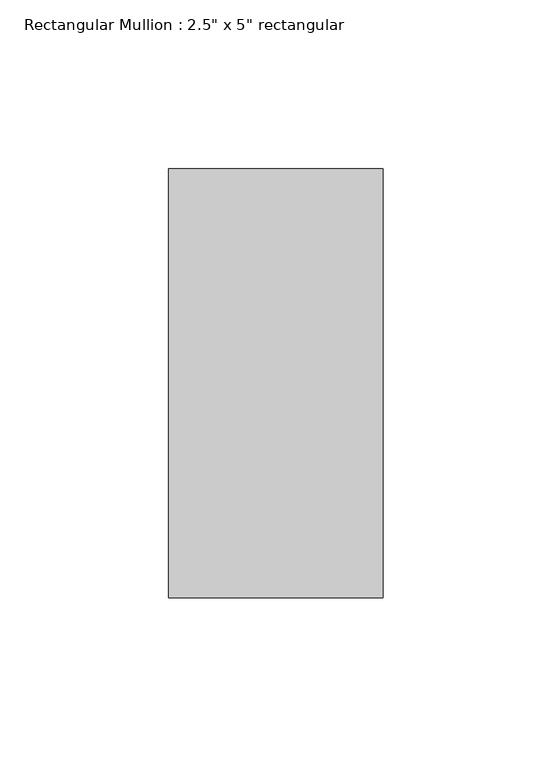
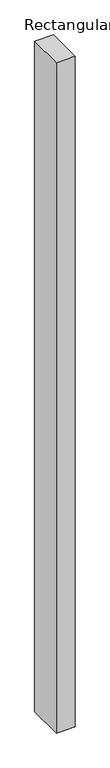
"""IFC4 building model written with IfcOpenShell, lengths in millimetres: member geometry."""

import ifcopenshell
import ifcopenshell.guid

model = None  # the IFC model being written
_history = None  # IfcOwnerHistory: only IFC2X3 demands one
_inside = {}  # id of a spatial element -> (the spatial element, [elements in it])
_under = {}  # id of a project, library or spatial element -> (it, [spatial elements below it])
_declared = {}  # id of a project -> (the project, [libraries it declares])
_typed = {}  # id of a type object -> (the type object, [elements of that type])
_made_of = {}  # id of a material, layer set ... -> (it, [elements and type objects made of it])


def new_model(schema):
    """Start an empty IFC model of exactly this schema.

    Asked for "IFC4X3", IfcOpenShell would pick the latest addendum, in which some entities
    have other attributes; the version numbers below select the first issue.
    IFC2X3 requires an IfcOwnerHistory on every rooted entity: one is made here for all.
    """
    global model, _history
    if schema == "IFC4X3":
        model = ifcopenshell.file(schema_version=(4, 3, 0, 0))
    else:
        model = ifcopenshell.file(schema=schema)
    _inside.clear()
    _under.clear()
    _declared.clear()
    _typed.clear()
    _made_of.clear()
    _history = None
    if model.schema == "IFC2X3":
        org = make("IfcOrganization", Name="unknown")
        user = make(
            "IfcPersonAndOrganization",
            ThePerson=make("IfcPerson", FamilyName="unknown"),
            TheOrganization=org,
        )
        app = make(
            "IfcApplication",
            ApplicationDeveloper=org,
            Version="unknown",
            ApplicationFullName="unknown",
            ApplicationIdentifier="unknown",
        )
        _history = make(
            "IfcOwnerHistory",
            OwningUser=user,
            OwningApplication=app,
            ChangeAction="ADDED",
            CreationDate=0,
        )
    return model


def make(cls, **values):
    """One entity of the class cls with the attributes given. An attribute that is None is left unset."""
    return model.create_entity(
        cls, **{name: value for name, value in values.items() if value is not None}
    )


def rooted(cls, **values):
    """An entity with a GlobalId (a new one), such as an element, a storey or a relation."""
    return make(cls, GlobalId=ifcopenshell.guid.new(), OwnerHistory=_history, **values)


def si_unit(unit_type, name, prefix=None):
    """IfcSIUnit, for example si_unit("LENGTHUNIT", "METRE", prefix="MILLI")."""
    return make("IfcSIUnit", UnitType=unit_type, Prefix=prefix, Name=name)


def assignment(units):
    """IfcUnitAssignment: the units of a project."""
    return None if units is None else make("IfcUnitAssignment", Units=units)


def point(xyz):
    """IfcCartesianPoint."""
    return None if xyz is None else make("IfcCartesianPoint", Coordinates=xyz)


def direction(xyz):
    """IfcDirection."""
    return None if xyz is None else make("IfcDirection", DirectionRatios=xyz)


def frame(location, z_axis=None, x_axis=None):
    """IfcAxis2Placement3D, a coordinate frame: its origin and axes. An axis left out is left unset."""
    return make(
        "IfcAxis2Placement3D",
        Location=point(location),
        Axis=direction(z_axis),
        RefDirection=direction(x_axis),
    )


def origin():
    """The frame at (0, 0, 0) with its axes left unset."""
    return frame((0.0, 0.0, 0.0))


def place(relative_to, where):
    """IfcLocalPlacement: puts the frame where relative to a parent placement (None: the world)."""
    return make(
        "IfcLocalPlacement", PlacementRelTo=relative_to, RelativePlacement=where
    )


def context(
    kind, dimensions, precision=None, world=None, true_north=None, identifier=None
):
    """IfcGeometricRepresentationContext, for example the 3D "Model" context."""
    return make(
        "IfcGeometricRepresentationContext",
        ContextIdentifier=identifier,
        ContextType=kind,
        CoordinateSpaceDimension=dimensions,
        Precision=precision,
        WorldCoordinateSystem=world,
        TrueNorth=true_north,
    )


def project(units=None, contexts=None):
    """IfcProject with its units and contexts."""
    return rooted(
        "IfcProject",
        Name="project",
        RepresentationContexts=contexts,
        UnitsInContext=assignment(units),
    )


def spatial(cls, under=None, at=None, **own):
    """A site, building, storey or space (cls), placed at a placement, below another one or the project."""
    s = rooted(cls, ObjectPlacement=at, **own)
    if under is not None:
        _under.setdefault(under.id(), (under, []))[1].append(s)
    return s


def polyline(points):
    """IfcPolyline through the points."""
    return make("IfcPolyline", Points=[point(p) for p in points])


def outline(outer, holes=None, kind="AREA"):
    """IfcArbitraryClosedProfileDef: a profile drawn as a closed curve; with holes, ...WithVoids."""
    if holes is None:
        return make("IfcArbitraryClosedProfileDef", ProfileType=kind, OuterCurve=outer)
    return make(
        "IfcArbitraryProfileDefWithVoids",
        ProfileType=kind,
        OuterCurve=outer,
        InnerCurves=holes,
    )


def extrude(swept, where, along, depth):
    """IfcExtrudedAreaSolid: the profile swept, set in the frame where, extruded along a direction by depth."""
    return make(
        "IfcExtrudedAreaSolid",
        SweptArea=swept,
        Position=where,
        ExtrudedDirection=direction(along),
        Depth=depth,
    )


def shape(context_of_items, identifier, shape_type, items):
    """IfcShapeRepresentation: the items that make up one representation, for example the "Body"."""
    return make(
        "IfcShapeRepresentation",
        ContextOfItems=context_of_items,
        RepresentationIdentifier=identifier,
        RepresentationType=shape_type,
        Items=items,
    )


def source(mapping_origin, context_of_items, identifier, shape_type, items):
    """IfcRepresentationMap: a shape defined once, which mapped items show again and again."""
    return make(
        "IfcRepresentationMap",
        MappingOrigin=mapping_origin,
        MappedRepresentation=shape(context_of_items, identifier, shape_type, items),
    )


def transform(
    local_origin,
    x_axis=None,
    y_axis=None,
    z_axis=None,
    scale=None,
    scale2=None,
    scale3=None,
    uniform=True,
):
    """IfcCartesianTransformationOperator3D, or its non-uniform kind. x_axis, y_axis, z_axis: its Axis1, 2, 3."""
    if uniform:
        return make(
            "IfcCartesianTransformationOperator3D",
            Axis1=direction(x_axis),
            Axis2=direction(y_axis),
            LocalOrigin=point(local_origin),
            Scale=scale,
            Axis3=direction(z_axis),
        )
    return make(
        "IfcCartesianTransformationOperator3DnonUniform",
        Axis1=direction(x_axis),
        Axis2=direction(y_axis),
        LocalOrigin=point(local_origin),
        Scale=scale,
        Axis3=direction(z_axis),
        Scale2=scale2,
        Scale3=scale3,
    )


def mapped(mapping_source, mapping_target):
    """IfcMappedItem: shows the shape of a source again, moved by a transform."""
    return make(
        "IfcMappedItem", MappingSource=mapping_source, MappingTarget=mapping_target
    )


def made_of(thing, what):
    """Note that an element or type object is made of a material, layer set ...; save() writes the relation."""
    if what is not None:
        _made_of.setdefault(what.id(), (what, []))[1].append(thing)
    return thing


def element(
    cls,
    number,
    at=None,
    inside=None,
    cuts=None,
    type_object=None,
    material=None,
    context=None,
    identifier="Body",
    shape_type=None,
    held_by="IfcProductDefinitionShape",
    body=None,
    shapes=None,
    **own,
):
    """One element of the class cls, such as IfcWall. Its Tag is "e" and its number.

    at: its placement. inside: the storey or other place that contains it. cuts: it is an
    opening in that element (IfcRelVoidsElement). A single representation is given by context,
    identifier, shape_type and body (its items); several are given by shapes. held_by: the class
    of the entity that holds the representations. save() writes the other relations.
    """
    e = rooted(cls, Tag="e%d" % number, ObjectPlacement=at, **own)
    if body is not None:
        shapes = [shape(context, identifier, shape_type, body)]
    if shapes is not None:
        e.Representation = make(held_by, Representations=shapes)
    if inside is not None:
        _inside.setdefault(inside.id(), (inside, []))[1].append(e)
    if cuts is not None:
        rooted(
            "IfcRelVoidsElement", RelatingBuildingElement=cuts, RelatedOpeningElement=e
        )
    if type_object is not None:
        _typed.setdefault(type_object.id(), (type_object, []))[1].append(e)
    return made_of(e, material)


def aggregate(whole, parts):
    """IfcRelAggregates: a whole, such as a stair, and the parts it consists of."""
    return rooted("IfcRelAggregates", RelatingObject=whole, RelatedObjects=parts)


def save(model, path):
    """Write the relations noted so far, then the file.

    IfcRelAggregates (storeys below a building ...), IfcRelContainedInSpatialStructure (elements
    in a storey), IfcRelDefinesByType, IfcRelAssociatesMaterial and IfcRelDeclares: one each for
    every whole, place, type object, material and project.
    """
    for whole, parts in _under.values():
        aggregate(whole, parts)
    for where, things in _inside.values():
        rooted(
            "IfcRelContainedInSpatialStructure",
            RelatedElements=things,
            RelatingStructure=where,
        )
    for kind, things in _typed.values():
        rooted("IfcRelDefinesByType", RelatedObjects=things, RelatingType=kind)
    for what, things in _made_of.values():
        rooted("IfcRelAssociatesMaterial", RelatedObjects=things, RelatingMaterial=what)
    for by, libraries in _declared.values():
        rooted("IfcRelDeclares", RelatingContext=by, RelatedDefinitions=libraries)
    model.write(path)


def member_5511fbbe(model_context):
    return source(origin(), model_context, "Body", "SweptSolid", [
        extrude(outline(polyline([(0.0, 63.5), (0.0, -63.5), (-63.5, -63.5), (-63.5, 63.5), (0.0, 63.5)])), frame((0.0, 0.0, -2398.3630718), z_axis=(0.0, 0.0, 1.0), x_axis=(1.0, 0.0, 0.0)), (0.0, 0.0, 1.0), 2398.3630718),
    ])


if __name__ == "__main__":
    model = new_model("IFC4")
    model_context = context("Model", 3, world=origin())
    ifc_project = project(units=[si_unit("LENGTHUNIT", "METRE", prefix="MILLI")], contexts=[model_context])
    site = spatial("IfcSite", under=ifc_project)
    building = spatial("IfcBuilding", under=site)
    placement = place(None, origin())
    member_shape = member_5511fbbe(model_context)
    element("IfcMember", 1, ObjectType="Rectangular Mullion : 2.5\" x 5\" rectangular", at=placement, inside=building, context=model_context, shape_type="MappedRepresentation", body=[
        mapped(member_shape, transform((0.0, 0.0, 0.0), x_axis=(1.0, 0.0, 0.0), y_axis=(0.0, 1.0, 0.0), z_axis=(0.0, 0.0, 1.0))),
    ])
    save(model, "model.ifc")

# Revit data of these elements
# Type "Rectangular Mullion : 2.5\" x 5\" rectangular"
#   built-in parameter 1007304 = 0.416667 (stored number, unit not read)
#   built-in parameter 1007301 = 0.104167 (stored number, unit not read)
#   built-in parameter 1007300 = 0.104167 (stored number, unit not read)
# Element 1 (IfcMember, "Rectangular Mullion : 2.5\" x 5\" rectangular")
#   Materials on its faces: "Aluminum"
# Materials
#   "Aluminum": class "Metal", colour RGB 247 247 247, transparency 0, Description = "Aluminum 6061", Cost = 0
